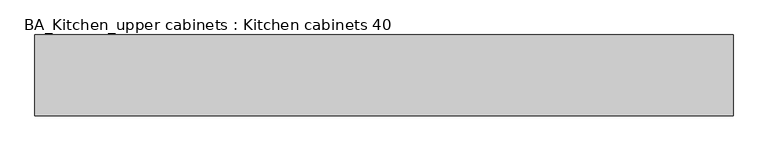
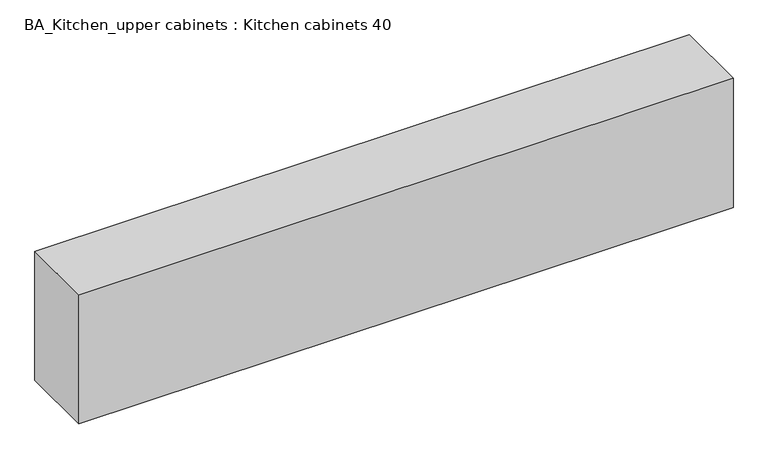
"""IFC4 building model written with IfcOpenShell, lengths in millimetres: furniture geometry, BA_Kitchen_upper cabinets : Kitchen cabinets 40."""

from ifc_helpers import new_model, si_unit, frame, origin, place, context, project, spatial, polyline, outline, extrude, source, transform, mapped, element, save


def ba_kitchen_upper_cabinets_kitchen_cabinets_40_4e662dbe(model_context):
    return source(origin(), model_context, "Body", "SweptSolid", [
        extrude(outline(polyline([(3450.0, 0.0), (0.0, 0.0), (0.0, 400.0), (3450.0, 400.0), (3450.0, 0.0)])), frame((0.0, 0.0, 1580.0), z_axis=(0.0, 0.0, 1.0), x_axis=(1.0, 0.0, 0.0)), (0.0, 0.0, 1.0), 720.0),
    ])


if __name__ == "__main__":
    model = new_model("IFC4")
    model_context = context("Model", 3, world=origin())
    ifc_project = project(units=[si_unit("LENGTHUNIT", "METRE", prefix="MILLI")], contexts=[model_context])
    site = spatial("IfcSite", under=ifc_project)
    building = spatial("IfcBuilding", under=site)
    placement = place(None, origin())
    ba_kitchen_upper_cabinets_kitchen_cabinets_40_shape = ba_kitchen_upper_cabinets_kitchen_cabinets_40_4e662dbe(model_context)
    element("IfcFurniture", 1, ObjectType="BA_Kitchen_upper cabinets : Kitchen cabinets 40", at=placement, inside=building, context=model_context, shape_type="MappedRepresentation", body=[
        mapped(ba_kitchen_upper_cabinets_kitchen_cabinets_40_shape, transform((0.0, 0.0, 0.0), x_axis=(1.0, 0.0, 0.0), y_axis=(0.0, 1.0, 0.0), z_axis=(0.0, 0.0, 1.0))),
    ])
    save(model, "model.ifc")

# Revit data of these elements
# Type "BA_Kitchen_upper cabinets : Kitchen cabinets 40"
#   built-in parameter 1001306 [instance default] = 4.85564 (stored number, unit not read)
#   Height [instance default] = 2300 mm
#   Depth = 400 mm
#   Default Elevation = 0
# Element 1 (IfcFurniture, "BA_Kitchen_upper cabinets : Kitchen cabinets 40")
#   built-in parameter 1001306 = 11.3189 (stored number, unit not read)
#   Materials on its faces: "Default"
# Materials
#   "Default": class "Generic", colour RGB 255 255 255, transparency 0, Cost = 0
